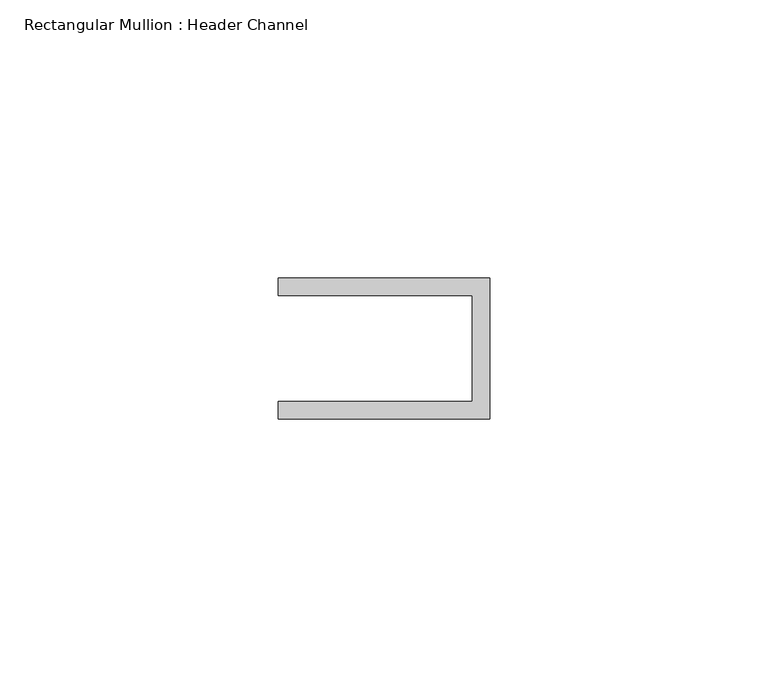
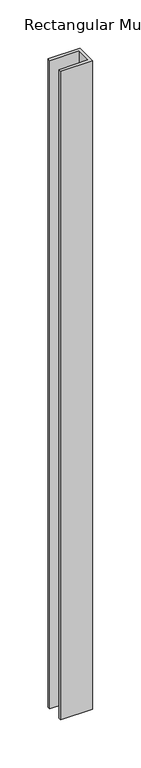
"""IFC4 building model written with IfcOpenShell, lengths in millimetres: member geometry, Rectangular Mullion : Header Channel."""

from ifc_helpers import new_model, si_unit, frame, origin, place, context, project, spatial, polyline, outline, extrude, source, transform, mapped, element, save


def rectangular_mullion_header_channel_dc101a94(model_context):
    return source(origin(), model_context, "Body", "SweptSolid", [
        extrude(outline(polyline([(0.0, -12.7), (-38.1, -12.7), (-38.1, -9.525), (-3.175, -9.525), (-3.175, 9.525), (-38.1, 9.525), (-38.1, 12.7), (0.0, 12.7), (0.0, -12.7)])), frame((0.0, 0.0, -817.5625), z_axis=(0.0, 0.0, 1.0), x_axis=(1.0, 0.0, 0.0)), (0.0, 0.0, 1.0), 817.5625),
    ])


if __name__ == "__main__":
    model = new_model("IFC4")
    model_context = context("Model", 3, world=origin())
    ifc_project = project(units=[si_unit("LENGTHUNIT", "METRE", prefix="MILLI")], contexts=[model_context])
    site = spatial("IfcSite", under=ifc_project)
    building = spatial("IfcBuilding", under=site)
    placement = place(None, origin())
    rectangular_mullion_header_channel_shape = rectangular_mullion_header_channel_dc101a94(model_context)
    element("IfcMember", 1, ObjectType="Rectangular Mullion : Header Channel", at=placement, inside=building, context=model_context, shape_type="MappedRepresentation", body=[
        mapped(rectangular_mullion_header_channel_shape, transform((0.0, 0.0, 0.0), x_axis=(1.0, 0.0, 0.0), y_axis=(0.0, 1.0, 0.0), z_axis=(0.0, 0.0, 1.0))),
    ])
    save(model, "model.ifc")

# Revit data of these elements
# Type "Rectangular Mullion : Header Channel"
#   built-in parameter 1007322 = 0.0833333 (stored number, unit not read)
#   built-in parameter 1007321 = -0.03125 (stored number, unit not read)
#   built-in parameter 1007320 = 0.0416667 (stored number, unit not read)
# Element 1 (IfcMember, "Rectangular Mullion : Header Channel")
#   Materials on its faces: "ALUM"
# Materials
#   "ALUM": class "Generic", colour RGB 157 157 157, transparency 0, Cost = 0
